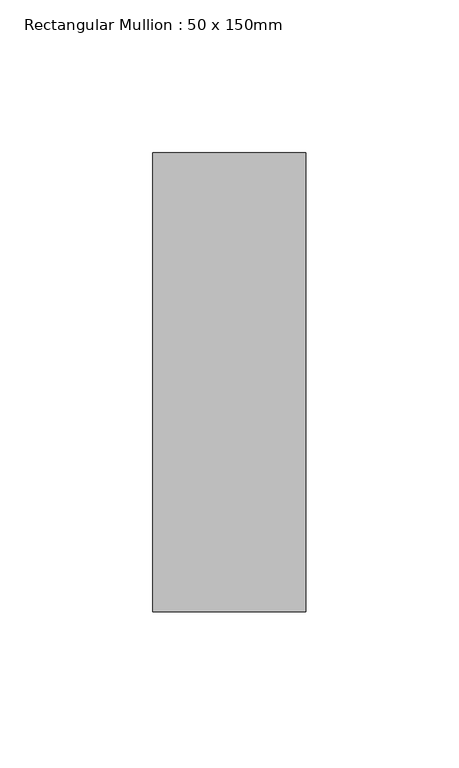
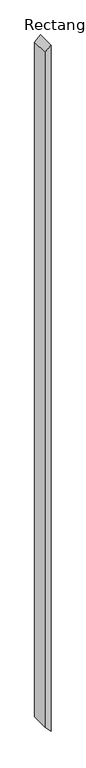
"""IFC4 building model written with IfcOpenShell, lengths in millimetres: member geometry, Rectangular Mullion : 50 x 150mm."""

from ifc_helpers import new_model, si_unit, frame, origin, place, context, project, spatial, polyline, outline, extrude, source, transform, mapped, element, save


def rectangular_mullion_50_x_150mm_f23ada83(model_context):
    return source(origin(), model_context, "Body", "SweptSolid", [
        extrude(outline(polyline([(0.0, 0.0), (-47.0734921, -50.0), (-6024.3583142, -50.0), (-6077.4667599, 0.0), (0.0, 0.0)])), frame((0.0, -75.0, 0.0), z_axis=(0.0, 1.0, 0.0), x_axis=(0.0, 0.0, 1.0)), (0.0, 0.0, 1.0), 150.0),
    ])


if __name__ == "__main__":
    model = new_model("IFC4")
    model_context = context("Model", 3, world=origin())
    ifc_project = project(units=[si_unit("LENGTHUNIT", "METRE", prefix="MILLI")], contexts=[model_context])
    site = spatial("IfcSite", under=ifc_project)
    building = spatial("IfcBuilding", under=site)
    placement = place(None, origin())
    rectangular_mullion_50_x_150mm_shape = rectangular_mullion_50_x_150mm_f23ada83(model_context)
    element("IfcMember", 1, ObjectType="Rectangular Mullion : 50 x 150mm", at=placement, inside=building, context=model_context, shape_type="MappedRepresentation", body=[
        mapped(rectangular_mullion_50_x_150mm_shape, transform((0.0, 0.0, 0.0), x_axis=(1.0, 0.0, 0.0), y_axis=(0.0, 1.0, 0.0), z_axis=(0.0, 0.0, 1.0))),
    ])
    save(model, "model.ifc")

# Revit data of these elements
# Type "Rectangular Mullion : 50 x 150mm"
#   built-in parameter 1007304 = 0.492126 (stored number, unit not read)
#   built-in parameter 1007301 = 0.082021 (stored number, unit not read)
#   built-in parameter 1007300 = 0.082021 (stored number, unit not read)
# Element 1 (IfcMember, "Rectangular Mullion : 50 x 150mm")
#   Materials on its faces: "Metal - Aluminium"
# Materials
#   "Metal - Aluminium": class "Metal", colour RGB 247 247 247, transparency 0
